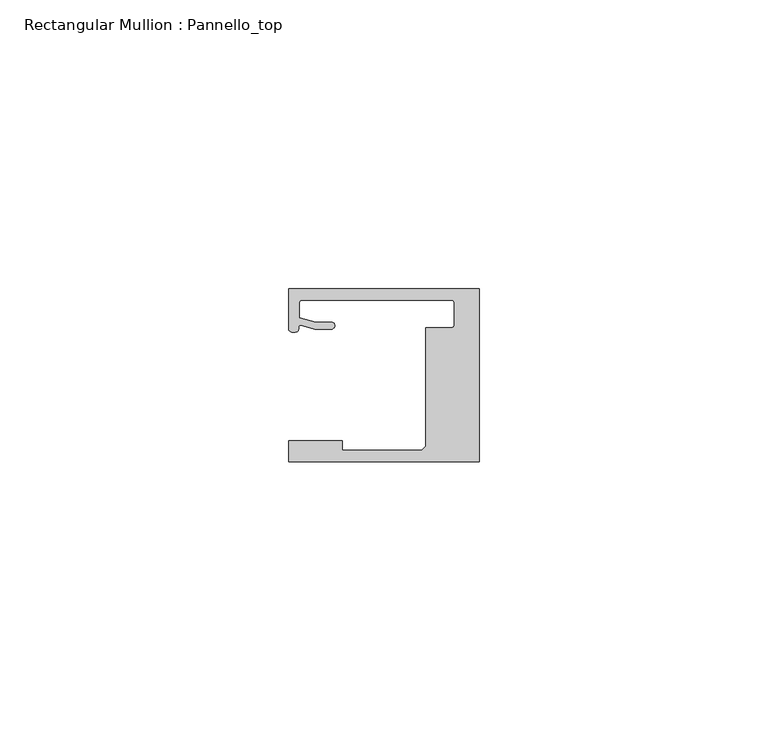
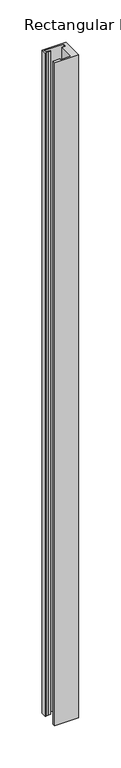
"""IFC4 building model written with IfcOpenShell, lengths in millimetres: member geometry, Rectangular Mullion : Pannello_top."""

from ifc_helpers import new_model, si_unit, frame, origin, place, context, project, spatial, polyline, circle_curve, source, transform, mapped, element, save
from ifc_brep_helpers import plane_surface, cylinder_surface, revolved_surface, extruded_surface, spline_curve, advanced_brep


def rectangular_mullion_pannello_top_78518063(model_context):
    return source(origin(), model_context, "Body", "AdvancedBrep", [
        advanced_brep(
        [(-33.0, -15.0, 0.0), (0.0, -15.0, 0.0), (0.0, 15.0, 0.0), (-33.0000135, 15.0, 0.0), (-33.0000135, 8.0000472, 0.0), (-30.9223017, 8.6490241, 0.0), (-28.4999305, 7.9999523, 0.0), (-25.59998, 7.9999523, 0.0), (-25.59998, 9.1999523, 0.0), (-28.3419477, 9.1999523, 0.0), (-31.19998, 9.9657591, 0.0), (-31.19998, 12.50001, 0.0), (-30.69998, 13.00001, 0.0), (-4.7999726, 13.00001, 0.0), (-4.2999726, 12.50001, 0.0), (-4.2999726, 8.7500595, 0.0), (-4.7999726, 8.2500595, 0.0), (-9.2999726, 8.2500595, 0.0), (-9.2999726, -12.2999849, 0.0), (-10.0000103, -13.0000004, 0.0), (-23.700041, -13.0000004, 0.0), (-23.700041, -11.3000004, 0.0), (-33.0, -11.3000004, 0.0), (-33.0, -15.0, -960.0), (-33.0, -11.3000004, -960.0), (-23.700041, -11.3000004, -960.0), (-23.700041, -13.0000004, -960.0), (-10.0000103, -13.0000004, -960.0), (-9.2999726, -12.2999849, -960.0), (-9.2999726, 8.2500595, -960.0), (-4.7999726, 8.2500595, -960.0), (-4.2999726, 8.7500595, -960.0), (-4.2999726, 12.50001, -960.0), (-4.7999726, 13.00001, -960.0), (-30.69998, 13.00001, -960.0), (-31.19998, 12.50001, -960.0), (-31.19998, 9.9657591, -960.0), (-28.3419477, 9.1999523, -960.0), (-25.59998, 9.1999523, -960.0), (-25.59998, 7.9999523, -960.0), (-28.4999305, 7.9999523, -960.0), (-30.9223017, 8.6490241, -960.0), (-33.0000135, 8.0000472, -960.0), (-33.0000135, 15.0, -960.0), (0.0, 15.0, -960.0), (0.0, -15.0, -960.0)],
        [
            (0, 1),
            (1, 2),
            (2, 3),
            (3, 4),
            (4, 5, spline_curve(3, [(-33.0000135, 8.0000472, 0.0), (-33.0000135, 7.457047519, 0.0), (-32.262327879, 7.456527435, 0.0), (-31.357433266, 7.563996614, 0.0), (-31.305645054, 7.690065204, 0.0), (-31.298563602, 8.366228555, 0.0), (-31.312054066, 8.717747958, 0.0), (-30.9223017, 8.6490241, 0.0)], [4, 2, 2, 4], [0.0, 0.0027053965905959043, 0.0058611956533709, 0.007702013405570312])),
            (5, 6),
            (6, 7),
            (7, 8, circle_curve(frame((-25.59998, 8.5999523, 0.0), z_axis=(0.0, 0.0, 1.0), x_axis=(0.0, 1.0, 0.0)), 0.6)),
            (8, 9),
            (9, 10),
            (10, 11),
            (11, 12, circle_curve(frame((-30.69998, 12.50001, 0.0), z_axis=(0.0, 0.0, -1.0), x_axis=(0.0, 1.0, 0.0)), 0.5)),
            (12, 13),
            (13, 14, circle_curve(frame((-4.7999726, 12.50001, 0.0), z_axis=(0.0, 0.0, -1.0), x_axis=(1.0, 0.0, 0.0)), 0.5)),
            (14, 15),
            (15, 16, circle_curve(frame((-4.7999726, 8.7500595, 0.0), z_axis=(0.0, 0.0, -1.0), x_axis=(0.0, -1.0, 0.0)), 0.5)),
            (16, 17),
            (17, 18),
            (18, 19),
            (19, 20),
            (20, 21),
            (21, 22),
            (22, 0),
            (23, 24),
            (24, 25),
            (25, 26),
            (26, 27),
            (27, 28),
            (28, 29),
            (29, 30),
            (30, 31, circle_curve(frame((-4.7999726, 8.7500595, -960.0), z_axis=(0.0, 0.0, 1.0), x_axis=(0.0, -1.0, 0.0)), 0.5)),
            (31, 32),
            (32, 33, circle_curve(frame((-4.7999726, 12.50001, -960.0), z_axis=(0.0, 0.0, 1.0), x_axis=(1.0, 0.0, 0.0)), 0.5)),
            (33, 34),
            (34, 35, circle_curve(frame((-30.69998, 12.50001, -960.0), z_axis=(0.0, 0.0, 1.0), x_axis=(0.0, 1.0, 0.0)), 0.5)),
            (35, 36),
            (36, 37),
            (37, 38),
            (38, 39, circle_curve(frame((-25.59998, 8.5999523, -960.0), z_axis=(0.0, 0.0, -1.0), x_axis=(0.0, 1.0, 0.0)), 0.6)),
            (39, 40),
            (40, 41),
            (41, 42, spline_curve(3, [(-30.9223017, 8.6490241, -960.0), (-31.312054066, 8.717747958, -960.0), (-31.298563602, 8.366228555, -960.0), (-31.305645054, 7.690065204, -960.0), (-31.357433266, 7.563996614, -960.0), (-32.262327879, 7.456527435, -960.0), (-33.0000135, 7.457047519, -960.0), (-33.0000135, 8.0000472, -960.0)], [4, 2, 2, 4], [0.0, 0.001840817752199412, 0.004996616814974408, 0.007702013405570312])),
            (42, 43),
            (43, 44),
            (44, 45),
            (45, 23),
            (0, 23),
            (45, 1),
            (44, 2),
            (43, 3),
            (42, 4),
            (41, 5),
            (40, 6),
            (39, 7),
            (38, 8),
            (37, 9),
            (36, 10),
            (35, 11),
            (34, 12),
            (33, 13),
            (32, 14),
            (31, 15),
            (30, 16),
            (29, 17),
            (28, 18),
            (27, 19),
            (26, 20),
            (25, 21),
            (24, 22),
        ],
        [
            plane_surface(frame((0.0, -36.2491502, 0.0), z_axis=(0.0, 0.0, 1.0), x_axis=(-1.0, 0.0, 0.0))),
            plane_surface(frame((0.0, -36.2491502, -960.0), z_axis=(0.0, 0.0, -1.0), x_axis=(-1.0, 0.0, 0.0))),
            plane_surface(frame((-33.0, -15.0, 0.0), z_axis=(0.0, -1.0, 0.0), x_axis=(0.0, 0.0, -1.0))),
            plane_surface(frame((0.0, -15.0, 0.0), z_axis=(1.0, 0.0, 0.0), x_axis=(0.0, 0.0, -1.0))),
            plane_surface(frame((0.0, 15.0, 0.0), z_axis=(0.0, 1.0, 0.0), x_axis=(0.0, 0.0, -1.0))),
            plane_surface(frame((-33.0000135, 15.0, 0.0), z_axis=(-1.0, 0.0, 0.0), x_axis=(0.0, 0.0, -1.0))),
            extruded_surface(spline_curve(3, [(-33.0000135, 8.0000472, -960.0), (-33.0000135, 7.457047519, -960.0), (-32.262327879, 7.456527435, -960.0), (-31.357433266, 7.563996614, -960.0), (-31.305645054, 7.690065204, -960.0), (-31.298563602, 8.366228555, -960.0), (-31.312054066, 8.717747958, -960.0), (-30.9223017, 8.6490241, -960.0)], [4, 2, 2, 4], [0.0, 0.0027053965905959043, 0.0058611956533709, 0.007702013405570312]), (0.0, 0.0, 960.0), 960.0),
            plane_surface(frame((-30.9223017, 8.6490241, 0.0), z_axis=(-0.25881883200192934, -0.9659258833891746, 0.0), x_axis=(0.0, 0.0, -1.0))),
            plane_surface(frame((-28.4999305, 7.9999523, 0.0), z_axis=(0.0, -1.0, 0.0), x_axis=(0.0, 0.0, -1.0))),
            cylinder_surface(frame((-25.59998, 8.5999523, 0.0), z_axis=(0.0, 0.0, 1.0), x_axis=(0.0, 1.0, 0.0)), 0.6),
            plane_surface(frame((-25.59998, 9.1999523, 0.0), z_axis=(0.0, 1.0, 0.0), x_axis=(0.0, 0.0, -1.0))),
            plane_surface(frame((-28.3419477, 9.1999523, 0.0), z_axis=(0.25881883204288636, 0.9659258833782002, 0.0), x_axis=(0.0, 0.0, -1.0))),
            plane_surface(frame((-31.19998, 9.9657591, 0.0), z_axis=(1.0, 0.0, 0.0), x_axis=(0.0, 0.0, -1.0))),
            revolved_surface(polyline([(-30.69998, 13.00001, -960.0), (-30.69998, 13.00001, 0.0)]), (-30.69998, 12.50001, 0.0), (0.0, 0.0, -1.0)),
            plane_surface(frame((-30.69998, 13.00001, 0.0), z_axis=(0.0, -1.0, 0.0), x_axis=(0.0, 0.0, -1.0))),
            revolved_surface(polyline([(-4.2999726, 12.50001, -960.0), (-4.2999726, 12.50001, 0.0)]), (-4.7999726, 12.50001, 0.0), (0.0, 0.0, -1.0)),
            plane_surface(frame((-4.2999726, 12.50001, 0.0), z_axis=(-1.0, 0.0, 0.0), x_axis=(0.0, 0.0, -1.0))),
            revolved_surface(polyline([(-4.7999726, 8.2500595, -960.0), (-4.7999726, 8.2500595, 0.0)]), (-4.7999726, 8.7500595, 0.0), (0.0, 0.0, -1.0)),
            plane_surface(frame((-4.7999726, 8.2500595, 0.0), z_axis=(0.0, 1.0, 0.0), x_axis=(0.0, 0.0, -1.0))),
            plane_surface(frame((-9.2999726, 8.2500595, 0.0), z_axis=(-1.0, 0.0, 0.0), x_axis=(0.0, 0.0, -1.0))),
            plane_surface(frame((-9.2999726, -12.2999849, 0.0), z_axis=(-0.7070955486277984, 0.7071180135668678, 0.0), x_axis=(0.0, 0.0, -1.0))),
            plane_surface(frame((-10.0000103, -13.0000004, 0.0), z_axis=(0.0, 1.0, 0.0), x_axis=(0.0, 0.0, -1.0))),
            plane_surface(frame((-23.700041, -13.0000004, 0.0), z_axis=(1.0, 0.0, 0.0), x_axis=(0.0, 0.0, -1.0))),
            plane_surface(frame((-23.700041, -11.3000004, 0.0), z_axis=(0.0, 1.0, 0.0), x_axis=(0.0, 0.0, -1.0))),
            plane_surface(frame((-33.0, -11.3000004, 0.0), z_axis=(-1.0, 0.0, 0.0), x_axis=(0.0, 0.0, -1.0))),
        ],
        [
            (0, [[1, 2, 3, 4, 5, 6, 7, 8, 9, 10, 11, 12, 13, 14, 15, 16, 17, 18, 19, 20, 21, 22, 23]]),
            (1, [[24, 25, 26, 27, 28, 29, 30, 31, 32, 33, 34, 35, 36, 37, 38, 39, 40, 41, 42, 43, 44, 45, 46]]),
            (2, [[-1, 47, -46, 48]]),
            (3, [[-2, -48, -45, 49]]),
            (4, [[-3, -49, -44, 50]]),
            (5, [[-4, -50, -43, 51]]),
            (6, [[-5, -51, -42, 52]]),
            (7, [[-6, -52, -41, 53]]),
            (8, [[-7, -53, -40, 54]]),
            (9, [[-8, -54, -39, 55]]),
            (10, [[-9, -55, -38, 56]]),
            (11, [[-10, -56, -37, 57]]),
            (12, [[-11, -57, -36, 58]]),
            (13, [[-12, -58, -35, 59]]),
            (14, [[-13, -59, -34, 60]]),
            (15, [[-14, -60, -33, 61]]),
            (16, [[-15, -61, -32, 62]]),
            (17, [[-16, -62, -31, 63]]),
            (18, [[-17, -63, -30, 64]]),
            (19, [[-18, -64, -29, 65]]),
            (20, [[-19, -65, -28, 66]]),
            (21, [[-20, -66, -27, 67]]),
            (22, [[-21, -67, -26, 68]]),
            (23, [[-22, -68, -25, 69]]),
            (24, [[-23, -69, -24, -47]]),
        ],
    ),
    ])


if __name__ == "__main__":
    model = new_model("IFC4")
    model_context = context("Model", 3, world=origin())
    ifc_project = project(units=[si_unit("LENGTHUNIT", "METRE", prefix="MILLI")], contexts=[model_context])
    site = spatial("IfcSite", under=ifc_project)
    building = spatial("IfcBuilding", under=site)
    placement = place(None, origin())
    rectangular_mullion_pannello_top_shape = rectangular_mullion_pannello_top_78518063(model_context)
    element("IfcMember", 1, ObjectType="Rectangular Mullion : Pannello_top", at=placement, inside=building, context=model_context, shape_type="MappedRepresentation", body=[
        mapped(rectangular_mullion_pannello_top_shape, transform((0.0, 0.0, 0.0), x_axis=(1.0, 0.0, 0.0), y_axis=(0.0, 1.0, 0.0), z_axis=(0.0, 0.0, 1.0))),
    ])
    save(model, "model.ifc")

# Revit data of these elements
# Type "Rectangular Mullion : Pannello_top"
#   built-in parameter 1007322 = 0.0984252 (stored number, unit not read)
#   built-in parameter 1007321 = 0 (stored number, unit not read)
#   built-in parameter 1007320 = 0.0305117 (stored number, unit not read)
